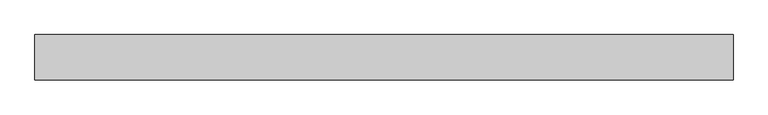
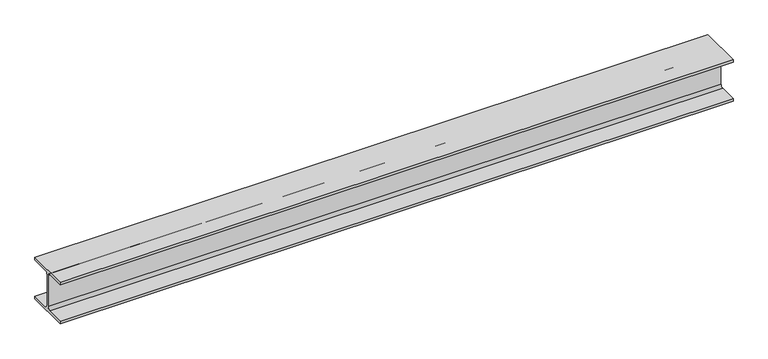
"""IFC4 building model written with IfcOpenShell, lengths in millimetres: beam geometry, 0912_Steel Framing_H-KSD3502 : H_SB_ASB_H-200x200x8x12."""

from ifc_helpers import new_model, si_unit, point, frame, frame_2d, origin, place, context, project, spatial, polyline, circle_curve, trimmed, segment, composite_curve, outline, extrude, source, transform, mapped, element, save


def beam_ad0691b1(model_context):
    return source(origin(), model_context, "Body", "SweptSolid", [
        extrude(outline(composite_curve([segment(polyline([(100.0, -88.0), (100.0, -100.0), (-100.0, -100.0), (-100.0, -88.0), (-17.0, -88.0)]), True, "CONTINUOUS"), segment(trimmed(circle_curve(frame_2d((-17.0, -75.0)), 13.0), [point((-17.0, -88.0))], [point((-4.0, -75.0))], True, "CARTESIAN"), True, "CONTINUOUS"), segment(polyline([(-4.0, -75.0), (-4.0, 75.0)]), True, "CONTINUOUS"), segment(trimmed(circle_curve(frame_2d((-17.0, 75.0)), 13.0), [point((-4.0, 75.0))], [point((-17.0, 88.0))], True, "CARTESIAN"), True, "CONTINUOUS"), segment(polyline([(-17.0, 88.0), (-100.0, 88.0), (-100.0, 100.0), (100.0, 100.0), (100.0, 88.0), (17.0, 88.0)]), True, "CONTINUOUS"), segment(trimmed(circle_curve(frame_2d((17.0, 75.0)), 13.0), [point((17.0, 88.0))], [point((4.0, 75.0))], True, "CARTESIAN"), True, "CONTINUOUS"), segment(polyline([(4.0, 75.0), (4.0, -75.0)]), True, "CONTINUOUS"), segment(trimmed(circle_curve(frame_2d((17.0, -75.0)), 13.0), [point((4.0, -75.0))], [point((17.0, -88.0))], True, "CARTESIAN"), True, "CONTINUOUS"), segment(polyline([(17.0, -88.0), (100.0, -88.0)]), True, "CONTINUOUS")], self_intersect=False)), frame((-1369.0394146, 0.0, 0.0), z_axis=(1.0, 0.0, 0.0), x_axis=(0.0, 1.0, 0.0)), (0.0, 0.0, 1.0), 3080.4153806),
    ])


if __name__ == "__main__":
    model = new_model("IFC4")
    model_context = context("Model", 3, world=origin())
    ifc_project = project(units=[si_unit("LENGTHUNIT", "METRE", prefix="MILLI")], contexts=[model_context])
    site = spatial("IfcSite", under=ifc_project)
    building = spatial("IfcBuilding", under=site)
    placement = place(None, origin())
    beam_shape = beam_ad0691b1(model_context)
    element("IfcBeam", 1, ObjectType="0912_Steel Framing_H-KSD3502 : H_SB_ASB_H-200x200x8x12", at=placement, inside=building, context=model_context, shape_type="MappedRepresentation", body=[
        mapped(beam_shape, transform((0.0, 0.0, 0.0), x_axis=(1.0, 0.0, 0.0), y_axis=(0.0, 1.0, 0.0), z_axis=(0.0, 0.0, 1.0))),
    ])
    save(model, "model.ifc")

# Revit data of these elements
# Type "0912_Steel Framing_H-KSD3502 : H_SB_ASB_H-200x200x8x12"
#   H_WM Code_1 = "S01AA002-00001 | Main Steel Structure Fabrication Work | Shelter/Building | Medium Steel - Standard (90KG/M>Weight≥30KG/M) | Material: (   )"
#   H_WM Code_2 = "S03AA028-00001 | Main Steel Structure Erection Work | Shelter/Building | Medium Steel (90KG/M>Weight≥30KG/M) | Material: (   )"
#   H_WM Code_3 = "S01AA010-00001 | Main Steel Structure Fabrication Work | Shelter/Building | Steel Painting/Coating | for Non-Fireproofed Steel Surface, Surface Preparation, Primer, Second & Final Coat | Material: (   )"
#   H_Q'ty Cal Type Tag = "SB-Q2"
#   Width = 20.0 cm
#   Web Thickness = 0.8 cm
#   Web Fillet = 1.3 cm
#   Warping Constant = 141000.0 cm⁶
#   W = 0
#   Torsional Moment of Inertia = 26.2485 cm⁴
#   Section Area = 63.53 cm²
#   Plastic Modulus weak axis = 244.0 cm³
#   Plastic Modulus strong axis = 525.0 cm³
#   Perimeter = 1.16 m²/m
#   Nominal Weight = 49.90 kgf/m
#   Moment of Inertia weak axis = 1600.00 cm⁴
#   Moment of Inertia strong axis = 4720.00 cm⁴
#   Height = 20.0 cm
#   Flange Thickness = 1.2 cm
#   Elastic Modulus weak axis = 160.0 cm³
#   Elastic Modulus strong axis = 472.0 cm³
#   Centroid Vertical = 10.0 cm
#   Centroid Horizontal = 10.0 cm
#   Ix = 47200000
#   Length [instance default] = 1.5240 m
#   Zx = 525000
#   b = 0.2000 m
#   h = 0.2000 m
#   r = 0.0130 m
#   s = 0.0080 m
#   t = 0.0120 m
#   A = 0.006353 m²
#   Structural Material [instance default] = Steel, 45-345
#   Assembly Code = ""
# Element 1 (IfcBeam, "0912_Steel Framing_H-KSD3502 : H_SB_ASB_H-200x200x8x12")
#   Structural Material = none
# Materials
#   "Steel, 45-345": class "Metal", colour RGB 189 187 185, transparency 0, Description = "Steel 345 MPa", Cost = 0
